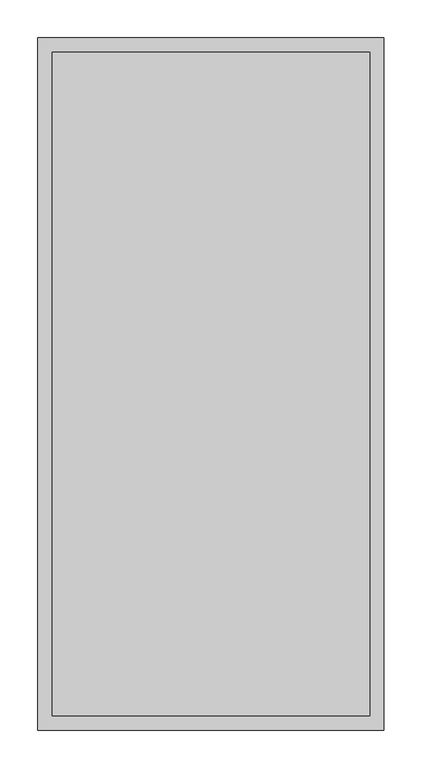
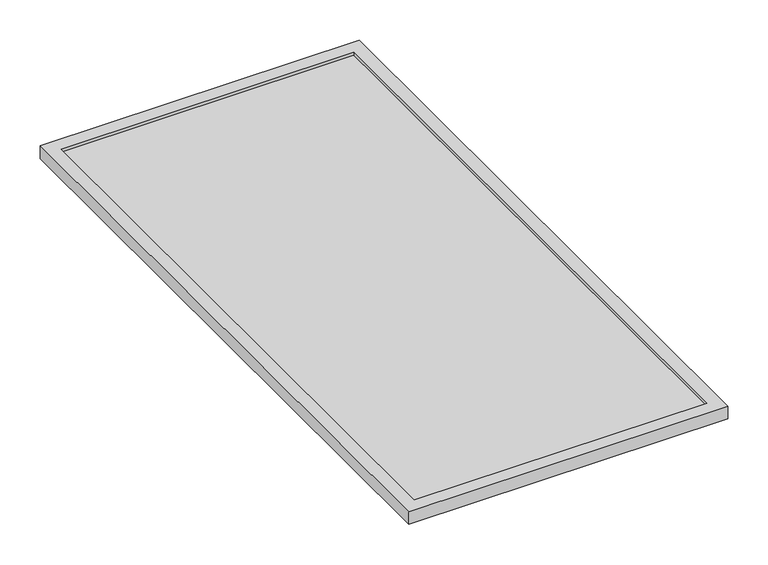
"""IFC4 building model written with IfcOpenShell, lengths in millimetres: proxy geometry, Bradley-Washroom_Accessories-Mirrors-780_Custom : Bradley-Washroom_Accessories-Mirrors-780_Custom."""

import ifcopenshell
import ifcopenshell.guid

model = None  # the IFC model being written
_history = None  # IfcOwnerHistory: only IFC2X3 demands one
_inside = {}  # id of a spatial element -> (the spatial element, [elements in it])
_under = {}  # id of a project, library or spatial element -> (it, [spatial elements below it])
_declared = {}  # id of a project -> (the project, [libraries it declares])
_typed = {}  # id of a type object -> (the type object, [elements of that type])
_made_of = {}  # id of a material, layer set ... -> (it, [elements and type objects made of it])


def new_model(schema):
    """Start an empty IFC model of exactly this schema.

    Asked for "IFC4X3", IfcOpenShell would pick the latest addendum, in which some entities
    have other attributes; the version numbers below select the first issue.
    IFC2X3 requires an IfcOwnerHistory on every rooted entity: one is made here for all.
    """
    global model, _history
    if schema == "IFC4X3":
        model = ifcopenshell.file(schema_version=(4, 3, 0, 0))
    else:
        model = ifcopenshell.file(schema=schema)
    _inside.clear()
    _under.clear()
    _declared.clear()
    _typed.clear()
    _made_of.clear()
    _history = None
    if model.schema == "IFC2X3":
        org = make("IfcOrganization", Name="unknown")
        user = make(
            "IfcPersonAndOrganization",
            ThePerson=make("IfcPerson", FamilyName="unknown"),
            TheOrganization=org,
        )
        app = make(
            "IfcApplication",
            ApplicationDeveloper=org,
            Version="unknown",
            ApplicationFullName="unknown",
            ApplicationIdentifier="unknown",
        )
        _history = make(
            "IfcOwnerHistory",
            OwningUser=user,
            OwningApplication=app,
            ChangeAction="ADDED",
            CreationDate=0,
        )
    return model


def make(cls, **values):
    """One entity of the class cls with the attributes given. An attribute that is None is left unset."""
    return model.create_entity(
        cls, **{name: value for name, value in values.items() if value is not None}
    )


def rooted(cls, **values):
    """An entity with a GlobalId (a new one), such as an element, a storey or a relation."""
    return make(cls, GlobalId=ifcopenshell.guid.new(), OwnerHistory=_history, **values)


def si_unit(unit_type, name, prefix=None):
    """IfcSIUnit, for example si_unit("LENGTHUNIT", "METRE", prefix="MILLI")."""
    return make("IfcSIUnit", UnitType=unit_type, Prefix=prefix, Name=name)


def assignment(units):
    """IfcUnitAssignment: the units of a project."""
    return None if units is None else make("IfcUnitAssignment", Units=units)


def point(xyz):
    """IfcCartesianPoint."""
    return None if xyz is None else make("IfcCartesianPoint", Coordinates=xyz)


def direction(xyz):
    """IfcDirection."""
    return None if xyz is None else make("IfcDirection", DirectionRatios=xyz)


def frame(location, z_axis=None, x_axis=None):
    """IfcAxis2Placement3D, a coordinate frame: its origin and axes. An axis left out is left unset."""
    return make(
        "IfcAxis2Placement3D",
        Location=point(location),
        Axis=direction(z_axis),
        RefDirection=direction(x_axis),
    )


def origin():
    """The frame at (0, 0, 0) with its axes left unset."""
    return frame((0.0, 0.0, 0.0))


def place(relative_to, where):
    """IfcLocalPlacement: puts the frame where relative to a parent placement (None: the world)."""
    return make(
        "IfcLocalPlacement", PlacementRelTo=relative_to, RelativePlacement=where
    )


def context(
    kind, dimensions, precision=None, world=None, true_north=None, identifier=None
):
    """IfcGeometricRepresentationContext, for example the 3D "Model" context."""
    return make(
        "IfcGeometricRepresentationContext",
        ContextIdentifier=identifier,
        ContextType=kind,
        CoordinateSpaceDimension=dimensions,
        Precision=precision,
        WorldCoordinateSystem=world,
        TrueNorth=true_north,
    )


def project(units=None, contexts=None):
    """IfcProject with its units and contexts."""
    return rooted(
        "IfcProject",
        Name="project",
        RepresentationContexts=contexts,
        UnitsInContext=assignment(units),
    )


def spatial(cls, under=None, at=None, **own):
    """A site, building, storey or space (cls), placed at a placement, below another one or the project."""
    s = rooted(cls, ObjectPlacement=at, **own)
    if under is not None:
        _under.setdefault(under.id(), (under, []))[1].append(s)
    return s


def polyline(points):
    """IfcPolyline through the points."""
    return make("IfcPolyline", Points=[point(p) for p in points])


def outline(outer, holes=None, kind="AREA"):
    """IfcArbitraryClosedProfileDef: a profile drawn as a closed curve; with holes, ...WithVoids."""
    if holes is None:
        return make("IfcArbitraryClosedProfileDef", ProfileType=kind, OuterCurve=outer)
    return make(
        "IfcArbitraryProfileDefWithVoids",
        ProfileType=kind,
        OuterCurve=outer,
        InnerCurves=holes,
    )


def extrude(swept, where, along, depth):
    """IfcExtrudedAreaSolid: the profile swept, set in the frame where, extruded along a direction by depth."""
    return make(
        "IfcExtrudedAreaSolid",
        SweptArea=swept,
        Position=where,
        ExtrudedDirection=direction(along),
        Depth=depth,
    )


def faces_of(points, faces, orient=None, outer=None):
    """IfcFace entities. A face is a list of loops; a loop is a list of indices into points, from 0.

    orient and outer hold one flag for each loop. By default every Orientation is true, the
    first loop of a face is its IfcFaceOuterBound and the others are IfcFaceBound.
    """
    made = []
    for i, loops in enumerate(faces):
        bounds = []
        for j, loop in enumerate(loops):
            is_outer = j == 0 if outer is None else outer[i][j]
            bounds.append(
                make(
                    "IfcFaceOuterBound" if is_outer else "IfcFaceBound",
                    Bound=make("IfcPolyLoop", Polygon=[points[k] for k in loop]),
                    Orientation=True if orient is None else orient[i][j],
                )
            )
        made.append(make("IfcFace", Bounds=bounds))
    return made


def faceted_brep(points, faces, orient=None, outer=None, voids=None):
    """IfcFacetedBrep: a solid bounded by flat faces; with voids (closed shells), ...WithVoids."""
    shared = [point(p) for p in points]
    hull = make("IfcClosedShell", CfsFaces=faces_of(shared, faces, orient, outer))
    if voids is None:
        return make("IfcFacetedBrep", Outer=hull)
    return make(
        "IfcFacetedBrepWithVoids",
        Outer=hull,
        Voids=[
            make(cls, CfsFaces=faces_of(shared, fs, o, b)) for cls, fs, o, b in voids
        ],
    )


def shape(context_of_items, identifier, shape_type, items):
    """IfcShapeRepresentation: the items that make up one representation, for example the "Body"."""
    return make(
        "IfcShapeRepresentation",
        ContextOfItems=context_of_items,
        RepresentationIdentifier=identifier,
        RepresentationType=shape_type,
        Items=items,
    )


def source(mapping_origin, context_of_items, identifier, shape_type, items):
    """IfcRepresentationMap: a shape defined once, which mapped items show again and again."""
    return make(
        "IfcRepresentationMap",
        MappingOrigin=mapping_origin,
        MappedRepresentation=shape(context_of_items, identifier, shape_type, items),
    )


def transform(
    local_origin,
    x_axis=None,
    y_axis=None,
    z_axis=None,
    scale=None,
    scale2=None,
    scale3=None,
    uniform=True,
):
    """IfcCartesianTransformationOperator3D, or its non-uniform kind. x_axis, y_axis, z_axis: its Axis1, 2, 3."""
    if uniform:
        return make(
            "IfcCartesianTransformationOperator3D",
            Axis1=direction(x_axis),
            Axis2=direction(y_axis),
            LocalOrigin=point(local_origin),
            Scale=scale,
            Axis3=direction(z_axis),
        )
    return make(
        "IfcCartesianTransformationOperator3DnonUniform",
        Axis1=direction(x_axis),
        Axis2=direction(y_axis),
        LocalOrigin=point(local_origin),
        Scale=scale,
        Axis3=direction(z_axis),
        Scale2=scale2,
        Scale3=scale3,
    )


def mapped(mapping_source, mapping_target):
    """IfcMappedItem: shows the shape of a source again, moved by a transform."""
    return make(
        "IfcMappedItem", MappingSource=mapping_source, MappingTarget=mapping_target
    )


def made_of(thing, what):
    """Note that an element or type object is made of a material, layer set ...; save() writes the relation."""
    if what is not None:
        _made_of.setdefault(what.id(), (what, []))[1].append(thing)
    return thing


def element(
    cls,
    number,
    at=None,
    inside=None,
    cuts=None,
    type_object=None,
    material=None,
    context=None,
    identifier="Body",
    shape_type=None,
    held_by="IfcProductDefinitionShape",
    body=None,
    shapes=None,
    **own,
):
    """One element of the class cls, such as IfcWall. Its Tag is "e" and its number.

    at: its placement. inside: the storey or other place that contains it. cuts: it is an
    opening in that element (IfcRelVoidsElement). A single representation is given by context,
    identifier, shape_type and body (its items); several are given by shapes. held_by: the class
    of the entity that holds the representations. save() writes the other relations.
    """
    e = rooted(cls, Tag="e%d" % number, ObjectPlacement=at, **own)
    if body is not None:
        shapes = [shape(context, identifier, shape_type, body)]
    if shapes is not None:
        e.Representation = make(held_by, Representations=shapes)
    if inside is not None:
        _inside.setdefault(inside.id(), (inside, []))[1].append(e)
    if cuts is not None:
        rooted(
            "IfcRelVoidsElement", RelatingBuildingElement=cuts, RelatedOpeningElement=e
        )
    if type_object is not None:
        _typed.setdefault(type_object.id(), (type_object, []))[1].append(e)
    return made_of(e, material)


def aggregate(whole, parts):
    """IfcRelAggregates: a whole, such as a stair, and the parts it consists of."""
    return rooted("IfcRelAggregates", RelatingObject=whole, RelatedObjects=parts)


def save(model, path):
    """Write the relations noted so far, then the file.

    IfcRelAggregates (storeys below a building ...), IfcRelContainedInSpatialStructure (elements
    in a storey), IfcRelDefinesByType, IfcRelAssociatesMaterial and IfcRelDeclares: one each for
    every whole, place, type object, material and project.
    """
    for whole, parts in _under.values():
        aggregate(whole, parts)
    for where, things in _inside.values():
        rooted(
            "IfcRelContainedInSpatialStructure",
            RelatedElements=things,
            RelatingStructure=where,
        )
    for kind, things in _typed.values():
        rooted("IfcRelDefinesByType", RelatedObjects=things, RelatingType=kind)
    for what, things in _made_of.values():
        rooted("IfcRelAssociatesMaterial", RelatedObjects=things, RelatingMaterial=what)
    for by, libraries in _declared.values():
        rooted("IfcRelDeclares", RelatingContext=by, RelatedDefinitions=libraries)
    model.write(path)


def specialty_equipment_075658ae(model_context):
    return source(origin(), model_context, "Body", "SolidModel", [
        extrude(outline(polyline([(209.55, -438.15), (-209.55, -438.15), (-209.55, 438.15), (209.55, 438.15), (209.55, -438.15)])), frame((0.0, 0.0, 9.525), z_axis=(0.0, 0.0, 1.0), x_axis=(1.0, 0.0, 0.0)), (0.0, 0.0, 1.0), 4.7625),
        faceted_brep([(228.6, -457.2, 19.05), (228.6, 457.2, 19.05), (-228.6, 457.2, 19.05), (-228.6, -457.2, 19.05), (-209.55, -438.15, 19.05), (-209.55, 438.15, 19.05), (209.55, 438.15, 19.05), (209.55, -438.15, 19.05), (228.6, -457.2, 0.0), (-228.6, -457.2, 0.0), (-228.6, 457.2, 0.0), (228.6, 457.2, 0.0), (209.55, -438.15, 9.525), (209.55, 438.15, 9.525), (-209.55, 438.15, 9.525), (-209.55, -438.15, 9.525)], [[[0, 1, 2, 3], [4, 5, 6, 7]], [[8, 9, 10, 11]], [[3, 9, 8, 0]], [[2, 10, 9, 3]], [[1, 11, 10, 2]], [[0, 8, 11, 1]], [[12, 13, 14, 15]], [[15, 4, 7, 12]], [[14, 5, 4, 15]], [[13, 6, 5, 14]], [[12, 7, 6, 13]]]),
    ])


if __name__ == "__main__":
    model = new_model("IFC4")
    model_context = context("Model", 3, world=origin())
    ifc_project = project(units=[si_unit("LENGTHUNIT", "METRE", prefix="MILLI")], contexts=[model_context])
    site = spatial("IfcSite", under=ifc_project)
    building = spatial("IfcBuilding", under=site)
    placement = place(None, origin())
    specialty_equipment_shape = specialty_equipment_075658ae(model_context)
    element("IfcBuildingElementProxy", 1, Name="Bradley-Washroom_Accessories-Mirrors-780_Custom : Bradley-Washroom_Accessories-Mirrors-780_Custom", ObjectType="Bradley-Washroom_Accessories-Mirrors-780_Custom : Bradley-Washroom_Accessories-Mirrors-780_Custom", at=placement, inside=building, context=model_context, shape_type="MappedRepresentation", body=[
        mapped(specialty_equipment_shape, transform((0.0, 0.0, 0.0), x_axis=(1.0, 0.0, 0.0), y_axis=(0.0, 1.0, 0.0), z_axis=(0.0, 0.0, 1.0))),
    ])
    save(model, "model.ifc")

# Revit data of these elements
# Project information
#   Project Issue Date = "07/20/2015"
#   Project Status = "Project Status"
#   Client Name = "Xcel"
#   Project Address = "Enter address here"
#   Project Name = "Sports Complex"
#   Project Number = "Project Number"
# Type "Bradley-Washroom_Accessories-Mirrors-780_Custom : Bradley-Washroom_Accessories-Mirrors-780_Custom"
#   Keynote = "M08831300.01"
#   Warranty Information = "Complete unit, excepting mirrors warranted for one year.\r\n Stainless steel mirror frames for fifteen years.\r\n Plate glass mirrors for fifteen years.\r\n This warranty does not cover installation or any other labor charges and does not apply to any units,\r\n which have been damaged by accident, abuse, improper installation, improper maintenance, or altered in any way."
#   Version = "1.0"
#   URL = "http://www.bradleycorp.com/"
#   Type Comments = "ERROR - If you are able to see this message you haven't loaded this  family correctly."
#   OmniClass Title = "Mirrors"
#   OmniClass Code = "23.40.95.17.17"
#   Modeling Code = ""
#   Model = "ERROR - If you are able to see this message you haven't loaded this  family correctly."
#   MasterFormat Title = "Commercial Toilet Accessories"
#   MasterFormat Number = "10 28 13. 13"
#   Manufacturer = "Bradley Corporation"
#   Industry Standards = "ASTM C 1036"
#   Fire Rating = "n/a"
#   Dimensional Limits [instance default] = "Either Width or Hight must be over 25\""
#   Description = "ERROR - If you are able to see this message you haven't loaded this  family correctly."
#   Copyright = "This Model Data is Property of Bradley Corporation"
#   Buy American Act = "Yes"
#   Assembly Code = "C1030900"
#   ADA Compliant = "Yes"
#   Width [instance default] = 1' - 6"
#   Total Width [instance default] = 1' - 6"
#   Total Height [instance default] = 3' - 0"
#   Height [instance default] = 3' - 0"
#   Depth [instance default] = 0' - 0 3/4"
#   Default Elevation = 3' - 4"
#   Reflective Material = Glass - Bradley Corp - BradEX - Polished Float Mirror
#   Frame Material = Bradley Corp Stainless Steel - Satin
# Element 1 (IfcBuildingElementProxy, "Bradley-Washroom_Accessories-Mirrors-780_Custom : Bradley-Washroom_Accessories-Mirrors-780_Custom")
#   Materials on its faces: "Bradley Corp Stainless Steel - Satin", "Glass - Bradley Corp - BradEX - Polished Float Mirror"
# Materials
#   "Glass - Bradley Corp - BradEX - Polished Float Mirror": class "Glass", colour RGB 221 230 232, transparency 0, Manufacturer = "Bradley Corporation", URL = "www.bradleycorp.com", Description = "Stainless Steel - Satin Finish", Cost = 0
#   "Bradley Corp Stainless Steel - Satin": class "Metal", colour RGB 189 187 185, transparency 0, Manufacturer = "Bradley Corporation", URL = "www.bradleycorp.com", Description = "Stainless Steel - Satin Finish", Cost = 0
